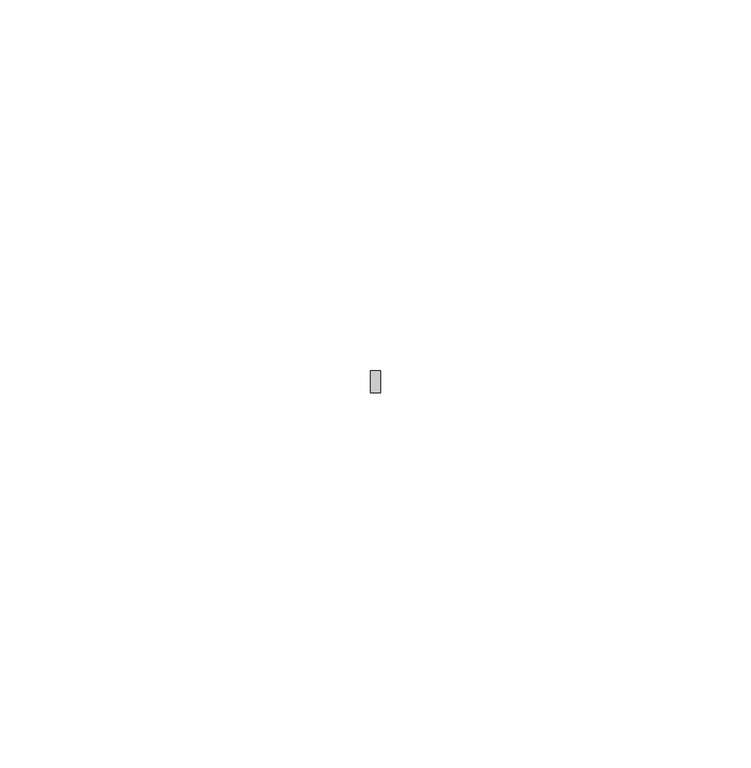
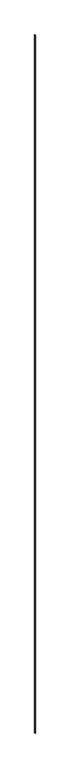
"""IFC4 building model written with IfcOpenShell, lengths in millimetres: proxy geometry, Generic Models 11:Generic Models 1:306267:Generic Models 1:306267 : Generic Models 11:Generic Models 1:306267:300405:Generic Models 1:306267:Generic Models 1:306267 : Generic Models 11:Generic Models 1:306267:300405 : Generic Models 11:Generic Models 1:306267:Generic Models 1:306267 : Generic Models 11:Generic Models 1:306267:300405:26 : Generic Models 11:Generic Models 1:306267:Generic Models 1:306267 : Generic Models 11:Generic Models 1:306267:300405:Generic Models 1:306267:Generic Models 1:306267 : Generic Models 11:Generic Models 1:306267:300405 : Generic Models 11:Generic Models 1:306267:Generic Models 1:306267 : Generic Models 11:Generic Models 1:306267:300405:300182."""

from ifc_helpers import new_model, si_unit, origin, origin_with_axes, place, context, project, spatial, polyline, outline, extrude, source, transform, mapped, element, save


def generic_models_49f1e31d(model_context):
    return source(origin(), model_context, "Body", "SweptSolid", [
        extrude(outline(polyline([(596182.8367239, -579013.3913841), (596184.1974915, -579013.3913841), (596184.1974915, -579016.3396517), (596182.8367239, -579016.3396517), (596182.8367239, -579013.3913841)])), origin_with_axes(), (0.0, 0.0, 1.0), 3689.35),
    ])


if __name__ == "__main__":
    model = new_model("IFC4")
    model_context = context("Model", 3, world=origin())
    ifc_project = project(units=[si_unit("LENGTHUNIT", "METRE", prefix="MILLI")], contexts=[model_context])
    site = spatial("IfcSite", under=ifc_project)
    building = spatial("IfcBuilding", under=site)
    placement = place(None, origin())
    generic_models_shape = generic_models_49f1e31d(model_context)
    element("IfcBuildingElementProxy", 1, Name="Generic Models 11:Generic Models 1:306267:Generic Models 1:306267 : Generic Models 11:Generic Models 1:306267:300405:Generic Models 1:306267:Generic Models 1:306267 : Generic Models 11:Generic Models 1:306267:300405 : Generic Models 11:Generic Models 1:306267:Generic Models 1:306267 : Generic Models 11:Generic Models 1:306267:300405:26 : Generic Models 11:Generic Models 1:306267:Generic Models 1:306267 : Generic Models 11:Generic Models 1:306267:300405:Generic Models 1:306267:Generic Models 1:306267 : Generic Models 11:Generic Models 1:306267:300405 : Generic Models 11:Generic Models 1:306267:Generic Models 1:306267 : Generic Models 11:Generic Models 1:306267:300405:300182", ObjectType="Generic Models 11:Generic Models 1:306267:Generic Models 1:306267 : Generic Models 11:Generic Models 1:306267:300405:Generic Models 1:306267:Generic Models 1:306267 : Generic Models 11:Generic Models 1:306267:300405 : Generic Models 11:Generic Models 1:306267:Generic Models 1:306267 : Generic Models 11:Generic Models 1:306267:300405:26 : Generic Models 11:Generic Models 1:306267:Generic Models 1:306267 : Generic Models 11:Generic Models 1:306267:300405:Generic Models 1:306267:Generic Models 1:306267 : Generic Models 11:Generic Models 1:306267:300405 : Generic Models 11:Generic Models 1:306267:Generic Models 1:306267 : Generic Models 11:Generic Models 1:306267:300405:300182", at=placement, inside=building, context=model_context, shape_type="MappedRepresentation", body=[
        mapped(generic_models_shape, transform((0.0, 0.0, 0.0), x_axis=(1.0, 0.0, 0.0), y_axis=(0.0, 1.0, 0.0), z_axis=(0.0, 0.0, 1.0))),
    ])
    save(model, "model.ifc")

# Revit data of these elements
# Type "Generic Models 11:Generic Models 1:306267:Generic Models 1:306267 : Generic Models 11:Generic Models 1:306267:300405:Generic Models 1:306267:Generic Models 1:306267 : Generic Models 11:Generic Models 1:306267:300405 : Generic Models 11:Generic Models 1:306267:Generic Models 1:306267 : Generic Models 11:Generic Models 1:306267:300405:26 : Generic Models 11:Generic Models 1:306267:Generic Models 1:306267 : Generic Models 11:Generic Models 1:306267:300405:Generic Models 1:306267:Generic Models 1:306267 : Generic Models 11:Generic Models 1:306267:300405 : Generic Models 11:Generic Models 1:306267:Generic Models 1:306267 : Generic Models 11:Generic Models 1:306267:300405:300182"
#   NameOverride = "Generic Models 11:Generic Models 1:306267:Generic Models 1:306267 : Generic Models 11:Generic Models 1:306267:300405:Generic Models 1:306267:Generic Models 1:306267 : Generic Models 11:Generic Models 1:306267:300405 : Generic Models 11:Generic Models 1:306267:Generic Models 1:306267 : Generic Models 11:Generic Models 1:306267:300405:300182"
#   ObjectTypeOverride = "Generic Models 1:306267:Generic Models 1:306267 : Generic Models 11:Generic Models 1:306267:300405 : Generic Models 11:Generic Models 1:306267:Generic Models 1:306267 : Generic Models 11:Generic Models 1:306267:300405"
#   Reference = "Generic Models 1"
#   Tag = "300182"
# Element 1 (IfcBuildingElementProxy, "Generic Models 11:Generic Models 1:306267:Generic Models 1:306267 : Generic Models 11:Generic Models 1:306267:300405:Generic Models 1:306267:Generic Models 1:306267 : Generic Models 11:Generic Models 1:306267:300405 : Generic Models 11:Generic Models 1:306267:Generic Models 1:306267 : Generic Models 11:Generic Models 1:306267:300405:26 : Generic Models 11:Generic Models 1:306267:Generic Models 1:306267 : Generic Models 11:Generic Models 1:306267:300405:Generic Models 1:306267:Generic Models 1:306267 : Generic Models 11:Generic Models 1:306267:300405 : Generic Models 11:Generic Models 1:306267:Generic Models 1:306267 : Generic Models 11:Generic Models 1:306267:300405:300182")
#   Materials on its faces: "UV STABLE WATER RESISTANT VAPOR PERMEABLE AIR BARRIER (WRB) - WRAP JAMBS/HEADERS - BLACK COLOR"
# Materials
#   "UV STABLE WATER RESISTANT VAPOR PERMEABLE AIR BARRIER (WRB) - WRAP JAMBS/HEADERS - BLACK COLOR": class "Generic", colour RGB 51 162 45, transparency 0, Description = "Polyethylene film membrane", Cost = 0
